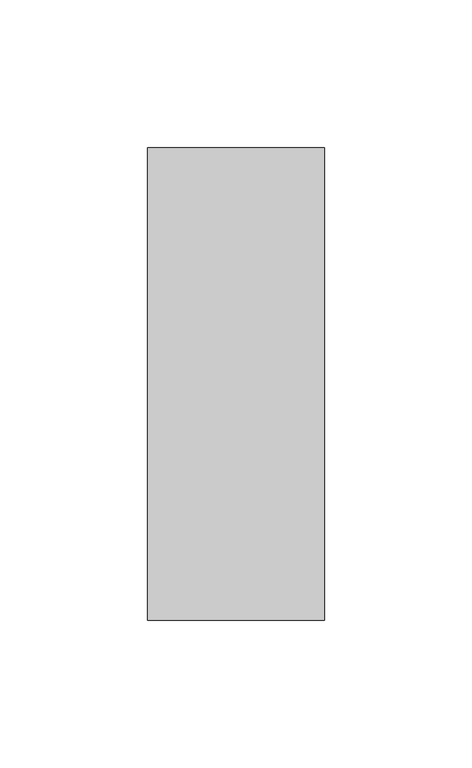
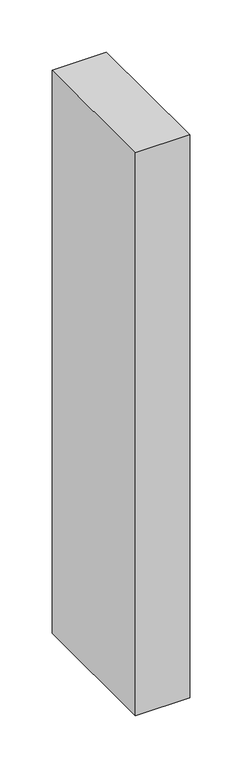
"""IFC4 building model written with IfcOpenShell, lengths in millimetres: column geometry, Madeira de lei-Coluna : Pontalete 6X16cm."""

from ifc_helpers import new_model, si_unit, frame, origin, place, context, project, spatial, polyline, outline, extrude, source, transform, mapped, element, save


def column_4db371bd(model_context):
    return source(origin(), model_context, "Body", "SweptSolid", [
        extrude(outline(polyline([(30.0, 80.0), (30.0, -80.0), (-30.0, -80.0), (-30.0, 80.0), (30.0, 80.0)])), frame((0.0, 0.0, 6710.0), z_axis=(0.0, 0.0, 1.0), x_axis=(1.0, 0.0, 0.0)), (0.0, 0.0, 1.0), 660.0),
    ])


if __name__ == "__main__":
    model = new_model("IFC4")
    model_context = context("Model", 3, world=origin())
    ifc_project = project(units=[si_unit("LENGTHUNIT", "METRE", prefix="MILLI")], contexts=[model_context])
    site = spatial("IfcSite", under=ifc_project)
    building = spatial("IfcBuilding", under=site)
    placement = place(None, origin())
    column_shape = column_4db371bd(model_context)
    element("IfcColumn", 1, ObjectType="Madeira de lei-Coluna : Pontalete 6X16cm", at=placement, inside=building, context=model_context, shape_type="MappedRepresentation", body=[
        mapped(column_shape, transform((0.0, 0.0, 0.0), x_axis=(1.0, 0.0, 0.0), y_axis=(0.0, 1.0, 0.0), z_axis=(0.0, 0.0, 1.0))),
    ])
    save(model, "model.ifc")

# Revit data of these elements
# Type "Madeira de lei-Coluna : Pontalete 6X16cm"
#   A = 0.01952 m²
#   b = 0.06 m
#   d = 0.16 m
#   Structural Material [instance default] = none
#   Assembly Code = ""
# Element 1 (IfcColumn, "Madeira de lei-Coluna : Pontalete 6X16cm")
#   Structural Material = .MADEIRAMENTO
#   Materials on its faces: ".MADEIRAMENTO"
# Materials
#   ".MADEIRAMENTO": class ".CC_MADEIRAS", colour RGB 212 179 113, transparency 0, Cost = 0
